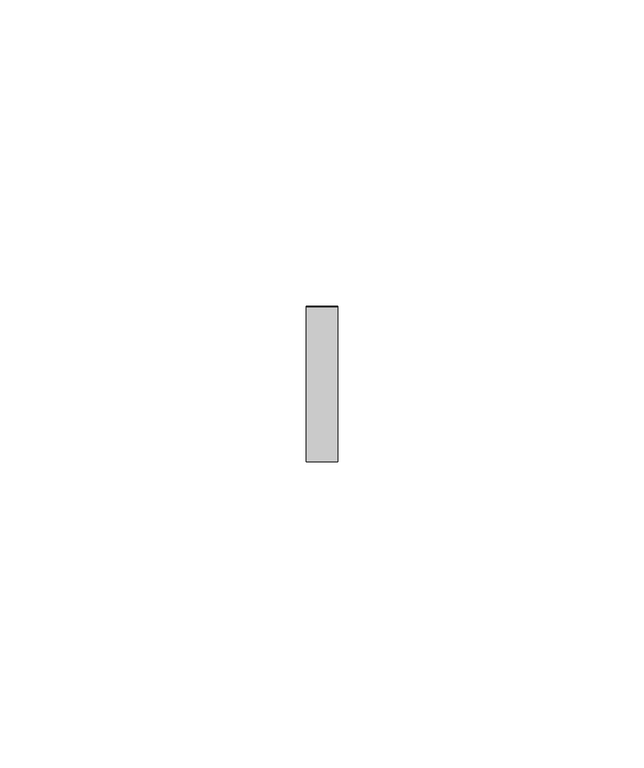
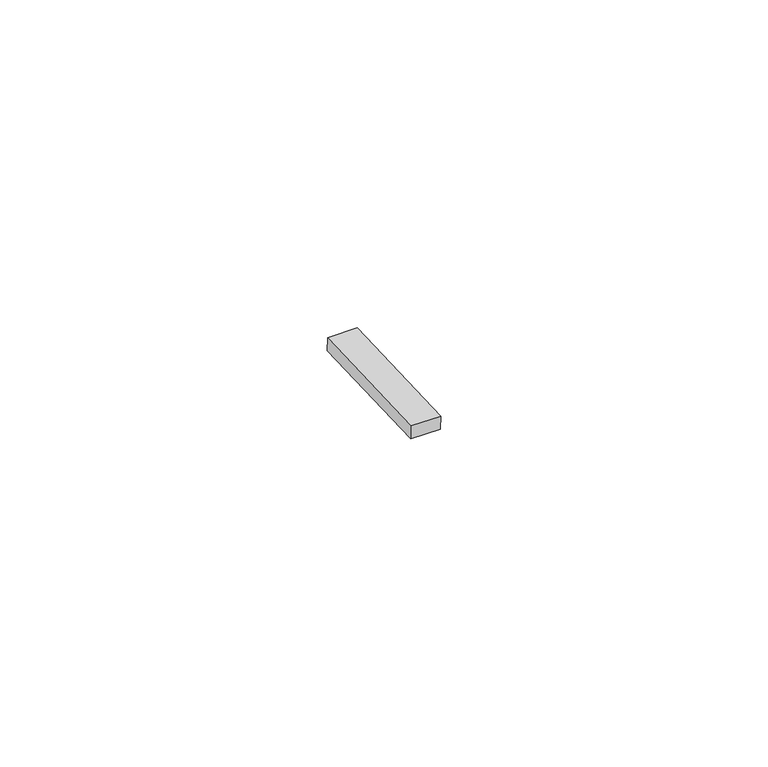
"""IFC4 building model written with IfcOpenShell, lengths in millimetres: proxy geometry, Inner panel:Inner panel:1:Inner panel:1 : Inner panel:Inner panel:300324:2:Inner panel:1:Inner panel:1 : Inner panel:Inner panel:300324:2 : Inner panel:Inner panel:1:Inner panel:1 : Inner panel:Inner panel:300324:300043:135 : Inner panel:Inner panel:1:Inner panel:1 : Inner panel:Inner panel:300324:2:Inner panel:1:Inner panel:1 : Inner panel:Inner panel:300324:2 : Inner panel:Inner panel:1:Inner panel:1 : Inner panel:Inner panel:300324:300043:308120."""

from ifc_helpers import new_model, si_unit, frame, origin, place, context, project, spatial, polyline, outline, extrude, source, transform, mapped, element, save


def generic_models_75be58b3(model_context):
    return source(origin(), model_context, "Body", "SweptSolid", [
        extrude(outline(polyline([(0.0, -25.3999999), (0.0, 0.0), (5.2138089, 0.0), (5.2138089, -25.3999999), (0.0, -25.3999999)])), frame((592717.395117, -568123.7593241, 8806.3160403), z_axis=(0.0, -0.041630544712223896, 0.9991330730923502), x_axis=(-1.0, 0.0, 0.0)), (0.0, 0.0, 1.0), 2.4763745),
    ])


if __name__ == "__main__":
    model = new_model("IFC4")
    model_context = context("Model", 3, world=origin())
    ifc_project = project(units=[si_unit("LENGTHUNIT", "METRE", prefix="MILLI")], contexts=[model_context])
    site = spatial("IfcSite", under=ifc_project)
    building = spatial("IfcBuilding", under=site)
    placement = place(None, origin())
    generic_models_shape = generic_models_75be58b3(model_context)
    element("IfcBuildingElementProxy", 1, Name="Inner panel:Inner panel:1:Inner panel:1 : Inner panel:Inner panel:300324:2:Inner panel:1:Inner panel:1 : Inner panel:Inner panel:300324:2 : Inner panel:Inner panel:1:Inner panel:1 : Inner panel:Inner panel:300324:300043:135 : Inner panel:Inner panel:1:Inner panel:1 : Inner panel:Inner panel:300324:2:Inner panel:1:Inner panel:1 : Inner panel:Inner panel:300324:2 : Inner panel:Inner panel:1:Inner panel:1 : Inner panel:Inner panel:300324:300043:308120", ObjectType="Inner panel:Inner panel:1:Inner panel:1 : Inner panel:Inner panel:300324:2:Inner panel:1:Inner panel:1 : Inner panel:Inner panel:300324:2 : Inner panel:Inner panel:1:Inner panel:1 : Inner panel:Inner panel:300324:300043:135 : Inner panel:Inner panel:1:Inner panel:1 : Inner panel:Inner panel:300324:2:Inner panel:1:Inner panel:1 : Inner panel:Inner panel:300324:2 : Inner panel:Inner panel:1:Inner panel:1 : Inner panel:Inner panel:300324:300043:308120", at=placement, inside=building, context=model_context, shape_type="MappedRepresentation", body=[
        mapped(generic_models_shape, transform((0.0, 0.0, 0.0), x_axis=(1.0, 0.0, 0.0), y_axis=(0.0, 1.0, 0.0), z_axis=(0.0, 0.0, 1.0))),
    ])
    save(model, "model.ifc")

# Revit data of these elements
# Type "Inner panel:Inner panel:1:Inner panel:1 : Inner panel:Inner panel:300324:2:Inner panel:1:Inner panel:1 : Inner panel:Inner panel:300324:2 : Inner panel:Inner panel:1:Inner panel:1 : Inner panel:Inner panel:300324:300043:135 : Inner panel:Inner panel:1:Inner panel:1 : Inner panel:Inner panel:300324:2:Inner panel:1:Inner panel:1 : Inner panel:Inner panel:300324:2 : Inner panel:Inner panel:1:Inner panel:1 : Inner panel:Inner panel:300324:300043:308120"
#   NameOverride = "Inner panel:Inner panel:1:Inner panel:1 : Inner panel:Inner panel:300324:2:Inner panel:1:Inner panel:1 : Inner panel:Inner panel:300324:2 : Inner panel:Inner panel:1:Inner panel:1 : Inner panel:Inner panel:300324:300043:308120"
#   ObjectTypeOverride = "Inner panel:1:Inner panel:1 : Inner panel:Inner panel:300324:2 : Inner panel:Inner panel:1:Inner panel:1 : Inner panel:Inner panel:300324:300043"
#   Reference = "Inner panel"
#   Tag = "308120"
# Element 1 (IfcBuildingElementProxy, "Inner panel:Inner panel:1:Inner panel:1 : Inner panel:Inner panel:300324:2:Inner panel:1:Inner panel:1 : Inner panel:Inner panel:300324:2 : Inner panel:Inner panel:1:Inner panel:1 : Inner panel:Inner panel:300324:300043:135 : Inner panel:Inner panel:1:Inner panel:1 : Inner panel:Inner panel:300324:2:Inner panel:1:Inner panel:1 : Inner panel:Inner panel:300324:2 : Inner panel:Inner panel:1:Inner panel:1 : Inner panel:Inner panel:300324:300043:308120")
#   Materials on its faces: "AT CLIP - 1\" WIDE NON ABSORBENT, WEATHER-RESISTANT NEOPRENE/EPDM/SBR FOAM"
# Materials
#   "AT CLIP - 1\" WIDE NON ABSORBENT, WEATHER-RESISTANT NEOPRENE/EPDM/SBR FOAM": class "Generic", colour RGB 85 85 85, transparency 0, Cost = 0
